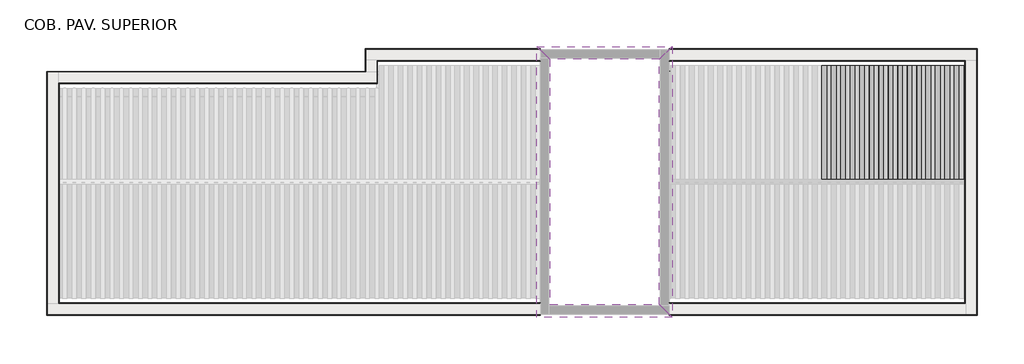
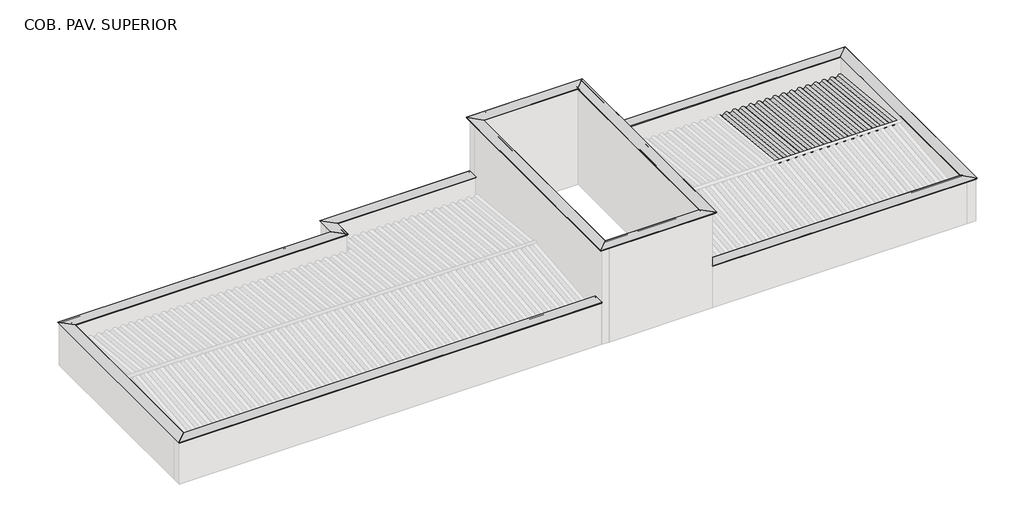
# One storey, part 7 of 7: 23 beams, 8 columns, 4 proxies.
"""IFC4 building model written with IfcOpenShell, lengths in millimetres."""

import ifcopenshell
import ifcopenshell.guid

model = None  # the IFC model being written
_history = None  # IfcOwnerHistory: only IFC2X3 demands one
_inside = {}  # id of a spatial element -> (the spatial element, [elements in it])
_under = {}  # id of a project, library or spatial element -> (it, [spatial elements below it])
_declared = {}  # id of a project -> (the project, [libraries it declares])
_typed = {}  # id of a type object -> (the type object, [elements of that type])
_made_of = {}  # id of a material, layer set ... -> (it, [elements and type objects made of it])


def new_model(schema):
    """Start an empty IFC model of exactly this schema.

    Asked for "IFC4X3", IfcOpenShell would pick the latest addendum, in which some entities
    have other attributes; the version numbers below select the first issue.
    IFC2X3 requires an IfcOwnerHistory on every rooted entity: one is made here for all.
    """
    global model, _history
    if schema == "IFC4X3":
        model = ifcopenshell.file(schema_version=(4, 3, 0, 0))
    else:
        model = ifcopenshell.file(schema=schema)
    _inside.clear()
    _under.clear()
    _declared.clear()
    _typed.clear()
    _made_of.clear()
    _history = None
    if model.schema == "IFC2X3":
        org = make("IfcOrganization", Name="unknown")
        user = make(
            "IfcPersonAndOrganization",
            ThePerson=make("IfcPerson", FamilyName="unknown"),
            TheOrganization=org,
        )
        app = make(
            "IfcApplication",
            ApplicationDeveloper=org,
            Version="unknown",
            ApplicationFullName="unknown",
            ApplicationIdentifier="unknown",
        )
        _history = make(
            "IfcOwnerHistory",
            OwningUser=user,
            OwningApplication=app,
            ChangeAction="ADDED",
            CreationDate=0,
        )
    return model


def make(cls, **values):
    """One entity of the class cls with the attributes given. An attribute that is None is left unset."""
    return model.create_entity(
        cls, **{name: value for name, value in values.items() if value is not None}
    )


def rooted(cls, **values):
    """An entity with a GlobalId (a new one), such as an element, a storey or a relation."""
    return make(cls, GlobalId=ifcopenshell.guid.new(), OwnerHistory=_history, **values)


def si_unit(unit_type, name, prefix=None):
    """IfcSIUnit, for example si_unit("LENGTHUNIT", "METRE", prefix="MILLI")."""
    return make("IfcSIUnit", UnitType=unit_type, Prefix=prefix, Name=name)


def assignment(units):
    """IfcUnitAssignment: the units of a project."""
    return None if units is None else make("IfcUnitAssignment", Units=units)


def point(xyz):
    """IfcCartesianPoint."""
    return None if xyz is None else make("IfcCartesianPoint", Coordinates=xyz)


def direction(xyz):
    """IfcDirection."""
    return None if xyz is None else make("IfcDirection", DirectionRatios=xyz)


def frame(location, z_axis=None, x_axis=None):
    """IfcAxis2Placement3D, a coordinate frame: its origin and axes. An axis left out is left unset."""
    return make(
        "IfcAxis2Placement3D",
        Location=point(location),
        Axis=direction(z_axis),
        RefDirection=direction(x_axis),
    )


def frame_2d(location, x_axis=None):
    """IfcAxis2Placement2D, a coordinate frame in the plane: its origin and x axis."""
    return make(
        "IfcAxis2Placement2D", Location=point(location), RefDirection=direction(x_axis)
    )


def origin():
    """The frame at (0, 0, 0) with its axes left unset."""
    return frame((0.0, 0.0, 0.0))


def place(relative_to, where):
    """IfcLocalPlacement: puts the frame where relative to a parent placement (None: the world)."""
    return make(
        "IfcLocalPlacement", PlacementRelTo=relative_to, RelativePlacement=where
    )


def context(
    kind, dimensions, precision=None, world=None, true_north=None, identifier=None
):
    """IfcGeometricRepresentationContext, for example the 3D "Model" context."""
    return make(
        "IfcGeometricRepresentationContext",
        ContextIdentifier=identifier,
        ContextType=kind,
        CoordinateSpaceDimension=dimensions,
        Precision=precision,
        WorldCoordinateSystem=world,
        TrueNorth=true_north,
    )


def project(units=None, contexts=None):
    """IfcProject with its units and contexts."""
    return rooted(
        "IfcProject",
        Name="project",
        RepresentationContexts=contexts,
        UnitsInContext=assignment(units),
    )


def spatial(cls, under=None, at=None, **own):
    """A site, building, storey or space (cls), placed at a placement, below another one or the project."""
    s = rooted(cls, ObjectPlacement=at, **own)
    if under is not None:
        _under.setdefault(under.id(), (under, []))[1].append(s)
    return s


def polyline(points):
    """IfcPolyline through the points."""
    return make("IfcPolyline", Points=[point(p) for p in points])


def circle_curve(where, radius):
    """IfcCircle in the frame where."""
    return make("IfcCircle", Position=where, Radius=radius)


def trimmed(basis, trim1, trim2, sense, master):
    """IfcTrimmedCurve: the piece of a basis curve between two trims."""
    return make(
        "IfcTrimmedCurve",
        BasisCurve=basis,
        Trim1=trim1,
        Trim2=trim2,
        SenseAgreement=sense,
        MasterRepresentation=master,
    )


def segment(curve, same_sense, transition):
    """IfcCompositeCurveSegment."""
    return make(
        "IfcCompositeCurveSegment",
        Transition=transition,
        SameSense=same_sense,
        ParentCurve=curve,
    )


def composite_curve(segments, self_intersect=None):
    """IfcCompositeCurve: segments joined end to end."""
    return make("IfcCompositeCurve", Segments=segments, SelfIntersect=self_intersect)


def outline(outer, holes=None, kind="AREA"):
    """IfcArbitraryClosedProfileDef: a profile drawn as a closed curve; with holes, ...WithVoids."""
    if holes is None:
        return make("IfcArbitraryClosedProfileDef", ProfileType=kind, OuterCurve=outer)
    return make(
        "IfcArbitraryProfileDefWithVoids",
        ProfileType=kind,
        OuterCurve=outer,
        InnerCurves=holes,
    )


def extrude(swept, where, along, depth):
    """IfcExtrudedAreaSolid: the profile swept, set in the frame where, extruded along a direction by depth."""
    return make(
        "IfcExtrudedAreaSolid",
        SweptArea=swept,
        Position=where,
        ExtrudedDirection=direction(along),
        Depth=depth,
    )


def faces_of(points, faces, orient=None, outer=None):
    """IfcFace entities. A face is a list of loops; a loop is a list of indices into points, from 0.

    orient and outer hold one flag for each loop. By default every Orientation is true, the
    first loop of a face is its IfcFaceOuterBound and the others are IfcFaceBound.
    """
    made = []
    for i, loops in enumerate(faces):
        bounds = []
        for j, loop in enumerate(loops):
            is_outer = j == 0 if outer is None else outer[i][j]
            bounds.append(
                make(
                    "IfcFaceOuterBound" if is_outer else "IfcFaceBound",
                    Bound=make("IfcPolyLoop", Polygon=[points[k] for k in loop]),
                    Orientation=True if orient is None else orient[i][j],
                )
            )
        made.append(make("IfcFace", Bounds=bounds))
    return made


def faceted_brep(points, faces, orient=None, outer=None, voids=None):
    """IfcFacetedBrep: a solid bounded by flat faces; with voids (closed shells), ...WithVoids."""
    shared = [point(p) for p in points]
    hull = make("IfcClosedShell", CfsFaces=faces_of(shared, faces, orient, outer))
    if voids is None:
        return make("IfcFacetedBrep", Outer=hull)
    return make(
        "IfcFacetedBrepWithVoids",
        Outer=hull,
        Voids=[
            make(cls, CfsFaces=faces_of(shared, fs, o, b)) for cls, fs, o, b in voids
        ],
    )


def shape(context_of_items, identifier, shape_type, items):
    """IfcShapeRepresentation: the items that make up one representation, for example the "Body"."""
    return make(
        "IfcShapeRepresentation",
        ContextOfItems=context_of_items,
        RepresentationIdentifier=identifier,
        RepresentationType=shape_type,
        Items=items,
    )


def source(mapping_origin, context_of_items, identifier, shape_type, items):
    """IfcRepresentationMap: a shape defined once, which mapped items show again and again."""
    return make(
        "IfcRepresentationMap",
        MappingOrigin=mapping_origin,
        MappedRepresentation=shape(context_of_items, identifier, shape_type, items),
    )


def transform(
    local_origin,
    x_axis=None,
    y_axis=None,
    z_axis=None,
    scale=None,
    scale2=None,
    scale3=None,
    uniform=True,
):
    """IfcCartesianTransformationOperator3D, or its non-uniform kind. x_axis, y_axis, z_axis: its Axis1, 2, 3."""
    if uniform:
        return make(
            "IfcCartesianTransformationOperator3D",
            Axis1=direction(x_axis),
            Axis2=direction(y_axis),
            LocalOrigin=point(local_origin),
            Scale=scale,
            Axis3=direction(z_axis),
        )
    return make(
        "IfcCartesianTransformationOperator3DnonUniform",
        Axis1=direction(x_axis),
        Axis2=direction(y_axis),
        LocalOrigin=point(local_origin),
        Scale=scale,
        Axis3=direction(z_axis),
        Scale2=scale2,
        Scale3=scale3,
    )


def mapped(mapping_source, mapping_target):
    """IfcMappedItem: shows the shape of a source again, moved by a transform."""
    return make(
        "IfcMappedItem", MappingSource=mapping_source, MappingTarget=mapping_target
    )


def made_of(thing, what):
    """Note that an element or type object is made of a material, layer set ...; save() writes the relation."""
    if what is not None:
        _made_of.setdefault(what.id(), (what, []))[1].append(thing)
    return thing


def element(
    cls,
    number,
    at=None,
    inside=None,
    cuts=None,
    type_object=None,
    material=None,
    context=None,
    identifier="Body",
    shape_type=None,
    held_by="IfcProductDefinitionShape",
    body=None,
    shapes=None,
    **own,
):
    """One element of the class cls, such as IfcWall. Its Tag is "e" and its number.

    at: its placement. inside: the storey or other place that contains it. cuts: it is an
    opening in that element (IfcRelVoidsElement). A single representation is given by context,
    identifier, shape_type and body (its items); several are given by shapes. held_by: the class
    of the entity that holds the representations. save() writes the other relations.
    """
    e = rooted(cls, Tag="e%d" % number, ObjectPlacement=at, **own)
    if body is not None:
        shapes = [shape(context, identifier, shape_type, body)]
    if shapes is not None:
        e.Representation = make(held_by, Representations=shapes)
    if inside is not None:
        _inside.setdefault(inside.id(), (inside, []))[1].append(e)
    if cuts is not None:
        rooted(
            "IfcRelVoidsElement", RelatingBuildingElement=cuts, RelatedOpeningElement=e
        )
    if type_object is not None:
        _typed.setdefault(type_object.id(), (type_object, []))[1].append(e)
    return made_of(e, material)


def aggregate(whole, parts):
    """IfcRelAggregates: a whole, such as a stair, and the parts it consists of."""
    return rooted("IfcRelAggregates", RelatingObject=whole, RelatedObjects=parts)


def save(model, path):
    """Write the relations noted so far, then the file.

    IfcRelAggregates (storeys below a building ...), IfcRelContainedInSpatialStructure (elements
    in a storey), IfcRelDefinesByType, IfcRelAssociatesMaterial and IfcRelDeclares: one each for
    every whole, place, type object, material and project.
    """
    for whole, parts in _under.values():
        aggregate(whole, parts)
    for where, things in _inside.values():
        rooted(
            "IfcRelContainedInSpatialStructure",
            RelatedElements=things,
            RelatingStructure=where,
        )
    for kind, things in _typed.values():
        rooted("IfcRelDefinesByType", RelatedObjects=things, RelatingType=kind)
    for what, things in _made_of.values():
        rooted("IfcRelAssociatesMaterial", RelatedObjects=things, RelatingMaterial=what)
    for by, libraries in _declared.values():
        rooted("IfcRelDeclares", RelatingContext=by, RelatedDefinitions=libraries)
    model.write(path)


def column_d505325c(model_context):
    return source(origin(), model_context, "Body", "SweptSolid", [
        extrude(outline(polyline([(30.0, 80.0), (30.0, -80.0), (-30.0, -80.0), (-30.0, 80.0), (30.0, 80.0)])), frame((0.0, 0.0, 6710.0), z_axis=(0.0, 0.0, 1.0), x_axis=(1.0, 0.0, 0.0)), (0.0, 0.0, 1.0), 750.0),
    ])


def column_4db371bd(model_context):
    return source(origin(), model_context, "Body", "SweptSolid", [
        extrude(outline(polyline([(30.0, 80.0), (30.0, -80.0), (-30.0, -80.0), (-30.0, 80.0), (30.0, 80.0)])), frame((0.0, 0.0, 6710.0), z_axis=(0.0, 0.0, 1.0), x_axis=(1.0, 0.0, 0.0)), (0.0, 0.0, 1.0), 660.0),
    ])


def column_d0cf395a(model_context):
    return source(origin(), model_context, "Body", "SweptSolid", [
        extrude(outline(polyline([(30.0, 80.0), (30.0, -80.0), (-30.0, -80.0), (-30.0, 80.0), (30.0, 80.0)])), frame((0.0, 0.0, 6710.0), z_axis=(0.0, 0.0, 1.0), x_axis=(1.0, 0.0, 0.0)), (0.0, 0.0, 1.0), 520.0),
    ])


model = new_model("IFC4")

# Units and contexts
model_context = context("Model", 3, world=origin())
ifc_project = project(units=[si_unit("LENGTHUNIT", "METRE", prefix="MILLI")], contexts=[model_context])

# Site, building, storey
site = spatial("IfcSite", under=ifc_project)
building = spatial("IfcBuilding", under=site)
storey = spatial("IfcBuildingStorey", under=building, Name="COB. PAV. SUPERIOR", Elevation=6650.0)

# Beams
placement = place(None, origin())
element("IfcBeam", 1, ObjectType="Madeira de lei : Berço 6x12cm", at=placement, inside=storey, context=model_context, shape_type="SweptSolid", body=[
    extrude(outline(polyline([(9090.718693, -7711.5607799), (9090.718693, -7831.5607799), (7090.718693, -7831.5607799), (7090.718693, -7711.5607799), (9090.718693, -7711.5607799)])), frame((0.0, 0.0, 6650.0), z_axis=(0.0, 0.0, 1.0), x_axis=(1.0, 0.0, 0.0)), (0.0, 0.0, 1.0), 60.0),
])
element("IfcBeam", 2, ObjectType="Madeira de lei : Berço 6x12cm", at=placement, inside=storey, context=model_context, shape_type="SweptSolid", body=[
    extrude(outline(polyline([(10730.718693, -7711.5607799), (10730.718693, -7831.5607799), (9090.718693, -7831.5607799), (9090.718693, -7711.5607799), (10730.718693, -7711.5607799)])), frame((0.0, 0.0, 6650.0), z_axis=(0.0, 0.0, 1.0), x_axis=(1.0, 0.0, 0.0)), (0.0, 0.0, 1.0), 60.0),
])
element("IfcBeam", 3, ObjectType="Madeira de lei : Berço 6x12cm", at=placement, inside=storey, context=model_context, shape_type="SweptSolid", body=[
    extrude(outline(polyline([(9089.7186924, -6319.8711004), (9089.7186924, -6439.8711004), (7089.7186936, -6439.8711004), (7089.7186936, -6319.8711004), (9089.7186924, -6319.8711004)])), frame((0.0, 0.0, 6650.0), z_axis=(0.0, 0.0, 1.0), x_axis=(1.0, 0.0, 0.0)), (0.0, 0.0, 1.0), 60.0),
])
element("IfcBeam", 4, ObjectType="Madeira de lei : Berço 6x12cm", at=placement, inside=storey, context=model_context, shape_type="SweptSolid", body=[
    extrude(outline(polyline([(10729.718693, -6319.8711004), (10729.718693, -6439.8711004), (9089.7186936, -6439.8711004), (9089.7186936, -6319.8711004), (10729.718693, -6319.8711004)])), frame((0.0, 0.0, 6650.0), z_axis=(0.0, 0.0, 1.0), x_axis=(1.0, 0.0, 0.0)), (0.0, 0.0, 1.0), 60.0),
])
element("IfcBeam", 5, ObjectType="Madeira de lei : Berço 6x12cm", at=placement, inside=storey, context=model_context, shape_type="SweptSolid", body=[
    extrude(outline(polyline([(5089.7186924, -4899.3026908), (5089.7186924, -5019.3026908), (3089.718693, -5019.3026908), (3089.718693, -4899.3026908), (5089.7186924, -4899.3026908)])), frame((0.0, 0.0, 6650.0), z_axis=(0.0, 0.0, 1.0), x_axis=(1.0, 0.0, 0.0)), (0.0, 0.0, 1.0), 60.0),
])
element("IfcBeam", 6, ObjectType="Madeira de lei : Berço 6x12cm", at=placement, inside=storey, context=model_context, shape_type="SweptSolid", body=[
    extrude(outline(polyline([(7089.7186924, -4899.3026908), (7089.7186924, -5019.3026908), (5089.7186936, -5019.3026908), (5089.7186936, -4899.3026908), (7089.7186924, -4899.3026908)])), frame((0.0, 0.0, 6650.0), z_axis=(0.0, 0.0, 1.0), x_axis=(1.0, 0.0, 0.0)), (0.0, 0.0, 1.0), 60.0),
])
element("IfcBeam", 7, ObjectType="Madeira de lei : Berço 6x12cm", at=placement, inside=storey, context=model_context, shape_type="SweptSolid", body=[
    extrude(outline(polyline([(9089.7186924, -4899.3026908), (9089.7186924, -5019.3026908), (7089.7186936, -5019.3026908), (7089.7186936, -4899.3026908), (9089.7186924, -4899.3026908)])), frame((0.0, 0.0, 6650.0), z_axis=(0.0, 0.0, 1.0), x_axis=(1.0, 0.0, 0.0)), (0.0, 0.0, 1.0), 60.0),
])
element("IfcBeam", 8, ObjectType="Madeira de lei : Berço 6x12cm", at=placement, inside=storey, context=model_context, shape_type="SweptSolid", body=[
    extrude(outline(polyline([(10729.718693, -4899.3026908), (10729.718693, -5019.3026908), (9089.7186936, -5019.3026908), (9089.7186936, -4899.3026908), (10729.718693, -4899.3026908)])), frame((0.0, 0.0, 6650.0), z_axis=(0.0, 0.0, 1.0), x_axis=(1.0, 0.0, 0.0)), (0.0, 0.0, 1.0), 60.0),
])
element("IfcBeam", 9, ObjectType="Telha Ondulada : Fibrocimento", at=placement, inside=storey, context=model_context, shape_type="SweptSolid", body=[
    extrude(outline(composite_curve([segment(trimmed(circle_curve(frame_2d((-58.7002978, -53.2060539)), 66.7939461), [point((-29.3501489, 6.7939461))], [point((-29.3501489, -113.2060539))], False, "CARTESIAN"), True, "CONTINUOUS"), segment(polyline([(-29.3501489, -113.2060539), (-31.5472154, -108.7146289)]), True, "CONTINUOUS"), segment(trimmed(circle_curve(frame_2d((-58.7002978, -53.2060539)), 61.7939461), [point((-31.5472154, -108.7146289))], [point((-31.5472154, 2.3025211))], True, "CARTESIAN"), True, "CONTINUOUS"), segment(trimmed(circle_curve(frame_2d((0.0, 66.7939461)), 71.7939461), [point((-31.5472154, 2.3025211))], [point((-31.5472154, 131.2853711))], False, "CARTESIAN"), True, "CONTINUOUS"), segment(polyline([(-31.5472154, 131.2853711), (-29.3501489, 126.7939461)]), True, "CONTINUOUS"), segment(trimmed(circle_curve(frame_2d((0.0, 66.7939461)), 66.7939461), [point((-29.3501489, 126.7939461))], [point((-29.3501489, 6.7939461))], True, "CARTESIAN"), True, "CONTINUOUS")], self_intersect=False)), frame((7168.1156257, -4759.1621575, 7394.5315886), z_axis=(0.0, -0.9950371902099893, 0.09950371902099778), x_axis=(0.0, 0.09950371902099778, 0.9950371902099893)), (0.0, 0.0, 1.0), 3017.2387654),
])
element("IfcBeam", 10, ObjectType="Telha Ondulada : Fibrocimento", at=placement, inside=storey, context=model_context, shape_type="SweptSolid", body=[
    extrude(outline(composite_curve([segment(trimmed(circle_curve(frame_2d((-58.7002978, -53.2060539)), 66.7939461), [point((-29.3501489, 6.7939461))], [point((-29.3501489, -113.2060539))], False, "CARTESIAN"), True, "CONTINUOUS"), segment(polyline([(-29.3501489, -113.2060539), (-31.5472154, -108.7146289)]), True, "CONTINUOUS"), segment(trimmed(circle_curve(frame_2d((-58.7002978, -53.2060539)), 61.7939461), [point((-31.5472154, -108.7146289))], [point((-31.5472154, 2.3025211))], True, "CARTESIAN"), True, "CONTINUOUS"), segment(trimmed(circle_curve(frame_2d((0.0, 66.7939461)), 71.7939461), [point((-31.5472154, 2.3025211))], [point((-31.5472154, 131.2853711))], False, "CARTESIAN"), True, "CONTINUOUS"), segment(polyline([(-31.5472154, 131.2853711), (-29.3501489, 126.7939461)]), True, "CONTINUOUS"), segment(trimmed(circle_curve(frame_2d((0.0, 66.7939461)), 66.7939461), [point((-29.3501489, 126.7939461))], [point((-29.3501489, 6.7939461))], True, "CARTESIAN"), True, "CONTINUOUS")], self_intersect=False)), frame((7412.6156257, -4759.1621575, 7394.5315886), z_axis=(0.0, -0.9950371902099893, 0.09950371902099776), x_axis=(0.0, 0.09950371902099776, 0.9950371902099893)), (0.0, 0.0, 1.0), 3017.2387654),
])
element("IfcBeam", 11, ObjectType="Telha Ondulada : Fibrocimento", at=placement, inside=storey, context=model_context, shape_type="SweptSolid", body=[
    extrude(outline(composite_curve([segment(trimmed(circle_curve(frame_2d((-58.7002978, -53.2060539)), 66.7939461), [point((-29.3501489, 6.7939461))], [point((-29.3501489, -113.2060539))], False, "CARTESIAN"), True, "CONTINUOUS"), segment(polyline([(-29.3501489, -113.2060539), (-31.5472154, -108.7146289)]), True, "CONTINUOUS"), segment(trimmed(circle_curve(frame_2d((-58.7002978, -53.2060539)), 61.7939461), [point((-31.5472154, -108.7146289))], [point((-31.5472154, 2.3025211))], True, "CARTESIAN"), True, "CONTINUOUS"), segment(trimmed(circle_curve(frame_2d((0.0, 66.7939461)), 71.7939461), [point((-31.5472154, 2.3025211))], [point((-31.5472154, 131.2853711))], False, "CARTESIAN"), True, "CONTINUOUS"), segment(polyline([(-31.5472154, 131.2853711), (-29.3501489, 126.7939461)]), True, "CONTINUOUS"), segment(trimmed(circle_curve(frame_2d((0.0, 66.7939461)), 66.7939461), [point((-29.3501489, 126.7939461))], [point((-29.3501489, 6.7939461))], True, "CARTESIAN"), True, "CONTINUOUS")], self_intersect=False)), frame((7657.1156257, -4759.1621575, 7394.5315886), z_axis=(0.0, -0.9950371902099893, 0.09950371902099775), x_axis=(0.0, 0.09950371902099775, 0.9950371902099893)), (0.0, 0.0, 1.0), 3017.2387654),
])
element("IfcBeam", 12, ObjectType="Telha Ondulada : Fibrocimento", at=placement, inside=storey, context=model_context, shape_type="SweptSolid", body=[
    extrude(outline(composite_curve([segment(trimmed(circle_curve(frame_2d((-58.7002978, -53.2060539)), 66.7939461), [point((-29.3501489, 6.7939461))], [point((-29.3501489, -113.2060539))], False, "CARTESIAN"), True, "CONTINUOUS"), segment(polyline([(-29.3501489, -113.2060539), (-31.5472154, -108.7146289)]), True, "CONTINUOUS"), segment(trimmed(circle_curve(frame_2d((-58.7002978, -53.2060539)), 61.7939461), [point((-31.5472154, -108.7146289))], [point((-31.5472154, 2.3025211))], True, "CARTESIAN"), True, "CONTINUOUS"), segment(trimmed(circle_curve(frame_2d((0.0, 66.7939461)), 71.7939461), [point((-31.5472154, 2.3025211))], [point((-31.5472154, 131.2853711))], False, "CARTESIAN"), True, "CONTINUOUS"), segment(polyline([(-31.5472154, 131.2853711), (-29.3501489, 126.7939461)]), True, "CONTINUOUS"), segment(trimmed(circle_curve(frame_2d((0.0, 66.7939461)), 66.7939461), [point((-29.3501489, 126.7939461))], [point((-29.3501489, 6.7939461))], True, "CARTESIAN"), True, "CONTINUOUS")], self_intersect=False)), frame((7901.6156257, -4759.1621575, 7394.5315886), z_axis=(0.0, -0.9950371902099893, 0.09950371902099778), x_axis=(0.0, 0.09950371902099778, 0.9950371902099893)), (0.0, 0.0, 1.0), 3017.2387654),
])
element("IfcBeam", 13, ObjectType="Telha Ondulada : Fibrocimento", at=placement, inside=storey, context=model_context, shape_type="SweptSolid", body=[
    extrude(outline(composite_curve([segment(trimmed(circle_curve(frame_2d((-58.7002978, -53.2060539)), 66.7939461), [point((-29.3501489, 6.7939461))], [point((-29.3501489, -113.2060539))], False, "CARTESIAN"), True, "CONTINUOUS"), segment(polyline([(-29.3501489, -113.2060539), (-31.5472154, -108.7146289)]), True, "CONTINUOUS"), segment(trimmed(circle_curve(frame_2d((-58.7002978, -53.2060539)), 61.7939461), [point((-31.5472154, -108.7146289))], [point((-31.5472154, 2.3025211))], True, "CARTESIAN"), True, "CONTINUOUS"), segment(trimmed(circle_curve(frame_2d((0.0, 66.7939461)), 71.7939461), [point((-31.5472154, 2.3025211))], [point((-31.5472154, 131.2853711))], False, "CARTESIAN"), True, "CONTINUOUS"), segment(polyline([(-31.5472154, 131.2853711), (-29.3501489, 126.7939461)]), True, "CONTINUOUS"), segment(trimmed(circle_curve(frame_2d((0.0, 66.7939461)), 66.7939461), [point((-29.3501489, 126.7939461))], [point((-29.3501489, 6.7939461))], True, "CARTESIAN"), True, "CONTINUOUS")], self_intersect=False)), frame((8146.1156257, -4759.1621575, 7394.5315886), z_axis=(0.0, -0.9950371902099893, 0.09950371902099776), x_axis=(0.0, 0.09950371902099776, 0.9950371902099893)), (0.0, 0.0, 1.0), 3017.2387654),
])
element("IfcBeam", 14, ObjectType="Telha Ondulada : Fibrocimento", at=placement, inside=storey, context=model_context, shape_type="SweptSolid", body=[
    extrude(outline(composite_curve([segment(trimmed(circle_curve(frame_2d((-58.7002978, -53.2060539)), 66.7939461), [point((-29.3501489, 6.7939461))], [point((-29.3501489, -113.2060539))], False, "CARTESIAN"), True, "CONTINUOUS"), segment(polyline([(-29.3501489, -113.2060539), (-31.5472154, -108.7146289)]), True, "CONTINUOUS"), segment(trimmed(circle_curve(frame_2d((-58.7002978, -53.2060539)), 61.7939461), [point((-31.5472154, -108.7146289))], [point((-31.5472154, 2.3025211))], True, "CARTESIAN"), True, "CONTINUOUS"), segment(trimmed(circle_curve(frame_2d((0.0, 66.7939461)), 71.7939461), [point((-31.5472154, 2.3025211))], [point((-31.5472154, 131.2853711))], False, "CARTESIAN"), True, "CONTINUOUS"), segment(polyline([(-31.5472154, 131.2853711), (-29.3501489, 126.7939461)]), True, "CONTINUOUS"), segment(trimmed(circle_curve(frame_2d((0.0, 66.7939461)), 66.7939461), [point((-29.3501489, 126.7939461))], [point((-29.3501489, 6.7939461))], True, "CARTESIAN"), True, "CONTINUOUS")], self_intersect=False)), frame((8390.6156257, -4759.1621575, 7394.5315886), z_axis=(0.0, -0.9950371902099893, 0.09950371902099776), x_axis=(0.0, 0.09950371902099776, 0.9950371902099893)), (0.0, 0.0, 1.0), 3017.2387654),
])
element("IfcBeam", 15, ObjectType="Telha Ondulada : Fibrocimento", at=placement, inside=storey, context=model_context, shape_type="SweptSolid", body=[
    extrude(outline(composite_curve([segment(trimmed(circle_curve(frame_2d((-58.7002978, -53.2060539)), 66.7939461), [point((-29.3501489, 6.7939461))], [point((-29.3501489, -113.2060539))], False, "CARTESIAN"), True, "CONTINUOUS"), segment(polyline([(-29.3501489, -113.2060539), (-31.5472154, -108.7146289)]), True, "CONTINUOUS"), segment(trimmed(circle_curve(frame_2d((-58.7002978, -53.2060539)), 61.7939461), [point((-31.5472154, -108.7146289))], [point((-31.5472154, 2.3025211))], True, "CARTESIAN"), True, "CONTINUOUS"), segment(trimmed(circle_curve(frame_2d((0.0, 66.7939461)), 71.7939461), [point((-31.5472154, 2.3025211))], [point((-31.5472154, 131.2853711))], False, "CARTESIAN"), True, "CONTINUOUS"), segment(polyline([(-31.5472154, 131.2853711), (-29.3501489, 126.7939461)]), True, "CONTINUOUS"), segment(trimmed(circle_curve(frame_2d((0.0, 66.7939461)), 66.7939461), [point((-29.3501489, 126.7939461))], [point((-29.3501489, 6.7939461))], True, "CARTESIAN"), True, "CONTINUOUS")], self_intersect=False)), frame((8635.1156257, -4759.1621575, 7394.5315886), z_axis=(0.0, -0.9950371902099893, 0.09950371902099778), x_axis=(0.0, 0.09950371902099778, 0.9950371902099893)), (0.0, 0.0, 1.0), 3017.2387654),
])
element("IfcBeam", 16, ObjectType="Telha Ondulada : Fibrocimento", at=placement, inside=storey, context=model_context, shape_type="SweptSolid", body=[
    extrude(outline(composite_curve([segment(trimmed(circle_curve(frame_2d((-58.7002978, -53.2060539)), 66.7939461), [point((-29.3501489, 6.7939461))], [point((-29.3501489, -113.2060539))], False, "CARTESIAN"), True, "CONTINUOUS"), segment(polyline([(-29.3501489, -113.2060539), (-31.5472154, -108.7146289)]), True, "CONTINUOUS"), segment(trimmed(circle_curve(frame_2d((-58.7002978, -53.2060539)), 61.7939461), [point((-31.5472154, -108.7146289))], [point((-31.5472154, 2.3025211))], True, "CARTESIAN"), True, "CONTINUOUS"), segment(trimmed(circle_curve(frame_2d((0.0, 66.7939461)), 71.7939461), [point((-31.5472154, 2.3025211))], [point((-31.5472154, 131.2853711))], False, "CARTESIAN"), True, "CONTINUOUS"), segment(polyline([(-31.5472154, 131.2853711), (-29.3501489, 126.7939461)]), True, "CONTINUOUS"), segment(trimmed(circle_curve(frame_2d((0.0, 66.7939461)), 66.7939461), [point((-29.3501489, 126.7939461))], [point((-29.3501489, 6.7939461))], True, "CARTESIAN"), True, "CONTINUOUS")], self_intersect=False)), frame((8879.6156257, -4759.1621575, 7394.5315886), z_axis=(0.0, -0.9950371902099893, 0.09950371902099778), x_axis=(0.0, 0.09950371902099778, 0.9950371902099893)), (0.0, 0.0, 1.0), 3017.2387654),
])
element("IfcBeam", 17, ObjectType="Telha Ondulada : Fibrocimento", at=placement, inside=storey, context=model_context, shape_type="SweptSolid", body=[
    extrude(outline(composite_curve([segment(trimmed(circle_curve(frame_2d((-58.7002978, -53.2060539)), 66.7939461), [point((-29.3501489, 6.7939461))], [point((-29.3501489, -113.2060539))], False, "CARTESIAN"), True, "CONTINUOUS"), segment(polyline([(-29.3501489, -113.2060539), (-31.5472154, -108.7146289)]), True, "CONTINUOUS"), segment(trimmed(circle_curve(frame_2d((-58.7002978, -53.2060539)), 61.7939461), [point((-31.5472154, -108.7146289))], [point((-31.5472154, 2.3025211))], True, "CARTESIAN"), True, "CONTINUOUS"), segment(trimmed(circle_curve(frame_2d((0.0, 66.7939461)), 71.7939461), [point((-31.5472154, 2.3025211))], [point((-31.5472154, 131.2853711))], False, "CARTESIAN"), True, "CONTINUOUS"), segment(polyline([(-31.5472154, 131.2853711), (-29.3501489, 126.7939461)]), True, "CONTINUOUS"), segment(trimmed(circle_curve(frame_2d((0.0, 66.7939461)), 66.7939461), [point((-29.3501489, 126.7939461))], [point((-29.3501489, 6.7939461))], True, "CARTESIAN"), True, "CONTINUOUS")], self_intersect=False)), frame((9124.1156257, -4759.1621575, 7394.5315886), z_axis=(0.0, -0.9950371902099893, 0.09950371902099776), x_axis=(0.0, 0.09950371902099776, 0.9950371902099893)), (0.0, 0.0, 1.0), 3017.2387654),
])
element("IfcBeam", 18, ObjectType="Telha Ondulada : Fibrocimento", at=placement, inside=storey, context=model_context, shape_type="SweptSolid", body=[
    extrude(outline(composite_curve([segment(trimmed(circle_curve(frame_2d((-58.7002978, -53.2060539)), 66.7939461), [point((-29.3501489, 6.7939461))], [point((-29.3501489, -113.2060539))], False, "CARTESIAN"), True, "CONTINUOUS"), segment(polyline([(-29.3501489, -113.2060539), (-31.5472154, -108.7146289)]), True, "CONTINUOUS"), segment(trimmed(circle_curve(frame_2d((-58.7002978, -53.2060539)), 61.7939461), [point((-31.5472154, -108.7146289))], [point((-31.5472154, 2.3025211))], True, "CARTESIAN"), True, "CONTINUOUS"), segment(trimmed(circle_curve(frame_2d((0.0, 66.7939461)), 71.7939461), [point((-31.5472154, 2.3025211))], [point((-31.5472154, 131.2853711))], False, "CARTESIAN"), True, "CONTINUOUS"), segment(polyline([(-31.5472154, 131.2853711), (-29.3501489, 126.7939461)]), True, "CONTINUOUS"), segment(trimmed(circle_curve(frame_2d((0.0, 66.7939461)), 66.7939461), [point((-29.3501489, 126.7939461))], [point((-29.3501489, 6.7939461))], True, "CARTESIAN"), True, "CONTINUOUS")], self_intersect=False)), frame((9368.6156257, -4759.1621575, 7394.5315886), z_axis=(0.0, -0.9950371902099893, 0.09950371902099776), x_axis=(0.0, 0.09950371902099776, 0.9950371902099893)), (0.0, 0.0, 1.0), 3017.2387654),
])
element("IfcBeam", 19, ObjectType="Telha Ondulada : Fibrocimento", at=placement, inside=storey, context=model_context, shape_type="SweptSolid", body=[
    extrude(outline(composite_curve([segment(trimmed(circle_curve(frame_2d((-58.7002978, -53.2060539)), 66.7939461), [point((-29.3501489, 6.7939461))], [point((-29.3501489, -113.2060539))], False, "CARTESIAN"), True, "CONTINUOUS"), segment(polyline([(-29.3501489, -113.2060539), (-31.5472154, -108.7146289)]), True, "CONTINUOUS"), segment(trimmed(circle_curve(frame_2d((-58.7002978, -53.2060539)), 61.7939461), [point((-31.5472154, -108.7146289))], [point((-31.5472154, 2.3025211))], True, "CARTESIAN"), True, "CONTINUOUS"), segment(trimmed(circle_curve(frame_2d((0.0, 66.7939461)), 71.7939461), [point((-31.5472154, 2.3025211))], [point((-31.5472154, 131.2853711))], False, "CARTESIAN"), True, "CONTINUOUS"), segment(polyline([(-31.5472154, 131.2853711), (-29.3501489, 126.7939461)]), True, "CONTINUOUS"), segment(trimmed(circle_curve(frame_2d((0.0, 66.7939461)), 66.7939461), [point((-29.3501489, 126.7939461))], [point((-29.3501489, 6.7939461))], True, "CARTESIAN"), True, "CONTINUOUS")], self_intersect=False)), frame((9613.1156257, -4759.1621575, 7394.5315886), z_axis=(0.0, -0.9950371902099893, 0.09950371902099775), x_axis=(0.0, 0.09950371902099775, 0.9950371902099893)), (0.0, 0.0, 1.0), 3017.2387654),
])
element("IfcBeam", 20, ObjectType="Telha Ondulada : Fibrocimento", at=placement, inside=storey, context=model_context, shape_type="SweptSolid", body=[
    extrude(outline(composite_curve([segment(trimmed(circle_curve(frame_2d((-58.7002978, -53.2060539)), 66.7939461), [point((-29.3501489, 6.7939461))], [point((-29.3501489, -113.2060539))], False, "CARTESIAN"), True, "CONTINUOUS"), segment(polyline([(-29.3501489, -113.2060539), (-31.5472154, -108.7146289)]), True, "CONTINUOUS"), segment(trimmed(circle_curve(frame_2d((-58.7002978, -53.2060539)), 61.7939461), [point((-31.5472154, -108.7146289))], [point((-31.5472154, 2.3025211))], True, "CARTESIAN"), True, "CONTINUOUS"), segment(trimmed(circle_curve(frame_2d((0.0, 66.7939461)), 71.7939461), [point((-31.5472154, 2.3025211))], [point((-31.5472154, 131.2853711))], False, "CARTESIAN"), True, "CONTINUOUS"), segment(polyline([(-31.5472154, 131.2853711), (-29.3501489, 126.7939461)]), True, "CONTINUOUS"), segment(trimmed(circle_curve(frame_2d((0.0, 66.7939461)), 66.7939461), [point((-29.3501489, 126.7939461))], [point((-29.3501489, 6.7939461))], True, "CARTESIAN"), True, "CONTINUOUS")], self_intersect=False)), frame((9857.6156257, -4759.1621575, 7394.5315886), z_axis=(0.0, -0.9950371902099893, 0.09950371902099778), x_axis=(0.0, 0.09950371902099778, 0.9950371902099893)), (0.0, 0.0, 1.0), 3017.2387654),
])
element("IfcBeam", 21, ObjectType="Telha Ondulada : Fibrocimento", at=placement, inside=storey, context=model_context, shape_type="SweptSolid", body=[
    extrude(outline(composite_curve([segment(trimmed(circle_curve(frame_2d((-58.7002978, -53.2060539)), 66.7939461), [point((-29.3501489, 6.7939461))], [point((-29.3501489, -113.2060539))], False, "CARTESIAN"), True, "CONTINUOUS"), segment(polyline([(-29.3501489, -113.2060539), (-31.5472154, -108.7146289)]), True, "CONTINUOUS"), segment(trimmed(circle_curve(frame_2d((-58.7002978, -53.2060539)), 61.7939461), [point((-31.5472154, -108.7146289))], [point((-31.5472154, 2.3025211))], True, "CARTESIAN"), True, "CONTINUOUS"), segment(trimmed(circle_curve(frame_2d((0.0, 66.7939461)), 71.7939461), [point((-31.5472154, 2.3025211))], [point((-31.5472154, 131.2853711))], False, "CARTESIAN"), True, "CONTINUOUS"), segment(polyline([(-31.5472154, 131.2853711), (-29.3501489, 126.7939461)]), True, "CONTINUOUS"), segment(trimmed(circle_curve(frame_2d((0.0, 66.7939461)), 66.7939461), [point((-29.3501489, 126.7939461))], [point((-29.3501489, 6.7939461))], True, "CARTESIAN"), True, "CONTINUOUS")], self_intersect=False)), frame((10102.1156257, -4759.1621575, 7394.5315886), z_axis=(0.0, -0.9950371902099893, 0.09950371902099776), x_axis=(0.0, 0.09950371902099776, 0.9950371902099893)), (0.0, 0.0, 1.0), 3017.2387654),
])
element("IfcBeam", 22, ObjectType="Telha Ondulada : Fibrocimento", at=placement, inside=storey, context=model_context, shape_type="SweptSolid", body=[
    extrude(outline(composite_curve([segment(trimmed(circle_curve(frame_2d((-58.7002978, -53.2060539)), 66.7939461), [point((-29.3501489, 6.7939461))], [point((-29.3501489, -113.2060539))], False, "CARTESIAN"), True, "CONTINUOUS"), segment(polyline([(-29.3501489, -113.2060539), (-31.5472154, -108.7146289)]), True, "CONTINUOUS"), segment(trimmed(circle_curve(frame_2d((-58.7002978, -53.2060539)), 61.7939461), [point((-31.5472154, -108.7146289))], [point((-31.5472154, 2.3025211))], True, "CARTESIAN"), True, "CONTINUOUS"), segment(trimmed(circle_curve(frame_2d((0.0, 66.7939461)), 71.7939461), [point((-31.5472154, 2.3025211))], [point((-31.5472154, 131.2853711))], False, "CARTESIAN"), True, "CONTINUOUS"), segment(polyline([(-31.5472154, 131.2853711), (-29.3501489, 126.7939461)]), True, "CONTINUOUS"), segment(trimmed(circle_curve(frame_2d((0.0, 66.7939461)), 66.7939461), [point((-29.3501489, 126.7939461))], [point((-29.3501489, 6.7939461))], True, "CARTESIAN"), True, "CONTINUOUS")], self_intersect=False)), frame((10346.6156257, -4759.1621575, 7394.5315886), z_axis=(0.0, -0.9950371902099893, 0.09950371902099776), x_axis=(0.0, 0.09950371902099776, 0.9950371902099893)), (0.0, 0.0, 1.0), 3017.2387654),
])
element("IfcBeam", 23, ObjectType="Telha Ondulada : Fibrocimento", at=placement, inside=storey, context=model_context, shape_type="SweptSolid", body=[
    extrude(outline(composite_curve([segment(trimmed(circle_curve(frame_2d((-58.7002978, -53.2060539)), 66.7939461), [point((-29.3501489, 6.7939461))], [point((-29.3501489, -113.2060539))], False, "CARTESIAN"), True, "CONTINUOUS"), segment(polyline([(-29.3501489, -113.2060539), (-31.5472154, -108.7146289)]), True, "CONTINUOUS"), segment(trimmed(circle_curve(frame_2d((-58.7002978, -53.2060539)), 61.7939461), [point((-31.5472154, -108.7146289))], [point((-31.5472154, 2.3025211))], True, "CARTESIAN"), True, "CONTINUOUS"), segment(trimmed(circle_curve(frame_2d((0.0, 66.7939461)), 71.7939461), [point((-31.5472154, 2.3025211))], [point((-31.5472154, 131.2853711))], False, "CARTESIAN"), True, "CONTINUOUS"), segment(polyline([(-31.5472154, 131.2853711), (-29.3501489, 126.7939461)]), True, "CONTINUOUS"), segment(trimmed(circle_curve(frame_2d((0.0, 66.7939461)), 66.7939461), [point((-29.3501489, 126.7939461))], [point((-29.3501489, 6.7939461))], True, "CARTESIAN"), True, "CONTINUOUS")], self_intersect=False)), frame((10591.1156257, -4759.1621575, 7394.5315886), z_axis=(0.0, -0.9950371902099893, 0.09950371902099778), x_axis=(0.0, 0.09950371902099778, 0.9950371902099893)), (0.0, 0.0, 1.0), 3017.2387654),
])

# Proxies
element("IfcBuildingElementProxy", 24, Name=".CC_RUFO_PINGADEIRA_27 cm", ObjectType=".CC_RUFO_PINGADEIRA_27 cm", at=placement, inside=storey, context=model_context, shape_type="Brep", body=[
    faceted_brep([(-4754.5024445, -4334.3488472, 7826.6820963), (-4747.4313766, -4341.419915, 7833.7531641), (-4747.4313766, -4341.419915, 7836.5815912), (-4754.0054581, -4334.8458336, 7830.0075098), (-4769.952748, -4318.8985437, 7860.0), (-4443.6098659, -4645.2414257, 7860.0), (-4459.5571559, -4629.2941358, 7830.0075098), (-4466.1312373, -4622.7200544, 7836.5815912), (-4466.1312373, -4622.7200544, 7833.7531641), (-4459.0601695, -4629.7911222, 7826.6820963), (-4440.281307, -4648.5699847, 7862.0), (-4773.281307, -4315.5699847, 7862.0), (-243.281307, -4334.3488472, 7826.6820963), (-243.281307, -4315.5699847, 7862.0), (-243.281307, -4648.5699847, 7862.0), (-243.281307, -4629.7911222, 7826.6820963), (-243.281307, -4622.7200544, 7833.7531641), (-243.281307, -4622.7200544, 7836.5815912), (-243.281307, -4629.2941358, 7830.0075098), (-243.281307, -4645.2414257, 7860.0), (-243.281307, -4318.8985437, 7860.0), (-243.281307, -4334.8458336, 7830.0075098), (-243.281307, -4341.419915, 7836.5815912), (-243.281307, -4341.419915, 7833.7531641)], [[[0, 1, 2, 3, 4, 5, 6, 7, 8, 9, 10, 11]], [[12, 13, 14, 15, 16, 17, 18, 19, 20, 21, 22, 23]], [[1, 0, 12, 23]], [[2, 1, 23, 22]], [[3, 2, 22, 21]], [[4, 3, 21, 20]], [[5, 4, 20, 19]], [[6, 5, 19, 18]], [[7, 6, 18, 17]], [[8, 7, 17, 16]], [[9, 8, 16, 15]], [[10, 9, 15, 14]], [[11, 10, 14, 13]], [[0, 11, 13, 12]]]),
    faceted_brep([(-4754.5024445, -4923.3488472, 7826.6820963), (-4747.4313766, -4930.419915, 7833.7531641), (-4747.4313766, -4930.419915, 7836.5815912), (-4754.0054581, -4923.8458336, 7830.0075098), (-4769.952748, -4907.8985437, 7860.0), (-4443.6098659, -5234.2414257, 7860.0), (-4459.5571559, -5218.2941358, 7830.0075098), (-4466.1312373, -5211.7200544, 7836.5815912), (-4466.1312373, -5211.7200544, 7833.7531641), (-4459.0601695, -5218.7911222, 7826.6820963), (-4440.281307, -5237.5699847, 7862.0), (-4773.281307, -4904.5699847, 7862.0), (-4754.5024445, -4334.3488472, 7826.6820963), (-4773.281307, -4315.5699847, 7862.0), (-4440.281307, -4648.5699847, 7862.0), (-4459.0601695, -4629.7911222, 7826.6820963), (-4466.1312373, -4622.7200544, 7833.7531641), (-4466.1312373, -4622.7200544, 7836.5815912), (-4459.5571559, -4629.2941358, 7830.0075098), (-4443.6098659, -4645.2414257, 7860.0), (-4769.952748, -4318.8985437, 7860.0), (-4754.0054581, -4334.8458336, 7830.0075098), (-4747.4313766, -4341.419915, 7836.5815912), (-4747.4313766, -4341.419915, 7833.7531641)], [[[0, 1, 2, 3, 4, 5, 6, 7, 8, 9, 10, 11]], [[12, 13, 14, 15, 16, 17, 18, 19, 20, 21, 22, 23]], [[1, 0, 12, 23]], [[2, 1, 23, 22]], [[3, 2, 22, 21]], [[4, 3, 21, 20]], [[5, 4, 20, 19]], [[6, 5, 19, 18]], [[7, 6, 18, 17]], [[8, 7, 17, 16]], [[9, 8, 16, 15]], [[10, 9, 15, 14]], [[11, 10, 14, 13]], [[0, 11, 13, 12]]]),
    faceted_brep([(-12982.5024444, -4923.3488472, 7826.6820963), (-12975.4313766, -4930.419915, 7833.7531641), (-12975.4313766, -4930.419915, 7836.5815912), (-12982.0054581, -4923.8458336, 7830.0075098), (-12997.952748, -4907.8985437, 7860.0), (-12671.6098659, -5234.2414257, 7860.0), (-12687.5571558, -5218.2941358, 7830.0075098), (-12694.1312373, -5211.7200544, 7836.5815912), (-12694.1312373, -5211.7200544, 7833.7531641), (-12687.0601695, -5218.7911222, 7826.6820963), (-12668.2813069, -5237.5699847, 7862.0), (-13001.2813069, -4904.5699847, 7862.0), (-4754.5024445, -4923.3488472, 7826.6820963), (-4773.281307, -4904.5699847, 7862.0), (-4440.281307, -5237.5699847, 7862.0), (-4459.0601695, -5218.7911222, 7826.6820963), (-4466.1312373, -5211.7200544, 7833.7531641), (-4466.1312373, -5211.7200544, 7836.5815912), (-4459.5571559, -5218.2941358, 7830.0075098), (-4443.6098659, -5234.2414257, 7860.0), (-4769.952748, -4907.8985437, 7860.0), (-4754.0054581, -4923.8458336, 7830.0075098), (-4747.4313766, -4930.419915, 7836.5815912), (-4747.4313766, -4930.419915, 7833.7531641)], [[[0, 1, 2, 3, 4, 5, 6, 7, 8, 9, 10, 11]], [[12, 13, 14, 15, 16, 17, 18, 19, 20, 21, 22, 23]], [[1, 0, 12, 23]], [[2, 1, 23, 22]], [[3, 2, 22, 21]], [[4, 3, 21, 20]], [[5, 4, 20, 19]], [[6, 5, 19, 18]], [[7, 6, 18, 17]], [[8, 7, 17, 16]], [[9, 8, 16, 15]], [[10, 9, 15, 14]], [[11, 10, 14, 13]], [[0, 11, 13, 12]]]),
    faceted_brep([(-12982.5024444, -11206.7911222, 7826.6820963), (-12975.4313766, -11199.7200544, 7833.7531641), (-12975.4313766, -11199.7200544, 7836.5815912), (-12982.0054581, -11206.2941358, 7830.0075098), (-12997.952748, -11222.2414257, 7860.0), (-12671.6098659, -10895.8985437, 7860.0), (-12687.5571558, -10911.8458336, 7830.0075098), (-12694.1312373, -10918.419915, 7836.5815912), (-12694.1312373, -10918.419915, 7833.7531641), (-12687.0601695, -10911.3488472, 7826.6820963), (-12668.2813069, -10892.5699847, 7862.0), (-13001.2813069, -11225.5699847, 7862.0), (-12982.5024444, -4923.3488472, 7826.6820963), (-13001.2813069, -4904.5699847, 7862.0), (-12668.2813069, -5237.5699847, 7862.0), (-12687.0601695, -5218.7911222, 7826.6820963), (-12694.1312373, -5211.7200544, 7833.7531641), (-12694.1312373, -5211.7200544, 7836.5815912), (-12687.5571558, -5218.2941358, 7830.0075098), (-12671.6098659, -5234.2414257, 7860.0), (-12997.952748, -4907.8985437, 7860.0), (-12982.0054581, -4923.8458336, 7830.0075098), (-12975.4313766, -4930.419915, 7836.5815912), (-12975.4313766, -4930.419915, 7833.7531641)], [[[0, 1, 2, 3, 4, 5, 6, 7, 8, 9, 10, 11]], [[12, 13, 14, 15, 16, 17, 18, 19, 20, 21, 22, 23]], [[1, 0, 12, 23]], [[2, 1, 23, 22]], [[3, 2, 22, 21]], [[4, 3, 21, 20]], [[5, 4, 20, 19]], [[6, 5, 19, 18]], [[7, 6, 18, 17]], [[8, 7, 17, 16]], [[9, 8, 16, 15]], [[10, 9, 15, 14]], [[11, 10, 14, 13]], [[0, 11, 13, 12]]]),
    faceted_brep([(-243.281307, -11206.7911222, 7826.6820963), (-243.281307, -11199.7200544, 7833.7531641), (-243.281307, -11199.7200544, 7836.5815912), (-243.281307, -11206.2941358, 7830.0075098), (-243.281307, -11222.2414257, 7860.0), (-243.281307, -10895.8985437, 7860.0), (-243.281307, -10911.8458336, 7830.0075098), (-243.281307, -10918.419915, 7836.5815912), (-243.281307, -10918.419915, 7833.7531641), (-243.281307, -10911.3488472, 7826.6820963), (-243.281307, -10892.5699847, 7862.0), (-243.281307, -11225.5699847, 7862.0), (-12982.5024444, -11206.7911222, 7826.6820963), (-13001.2813069, -11225.5699847, 7862.0), (-12668.2813069, -10892.5699847, 7862.0), (-12687.0601695, -10911.3488472, 7826.6820963), (-12694.1312373, -10918.419915, 7833.7531641), (-12694.1312373, -10918.419915, 7836.5815912), (-12687.5571558, -10911.8458336, 7830.0075098), (-12671.6098659, -10895.8985437, 7860.0), (-12997.952748, -11222.2414257, 7860.0), (-12982.0054581, -11206.2941358, 7830.0075098), (-12975.4313766, -11199.7200544, 7836.5815912), (-12975.4313766, -11199.7200544, 7833.7531641)], [[[0, 1, 2, 3, 4, 5, 6, 7, 8, 9, 10, 11]], [[12, 13, 14, 15, 16, 17, 18, 19, 20, 21, 22, 23]], [[1, 0, 12, 23]], [[2, 1, 23, 22]], [[3, 2, 22, 21]], [[4, 3, 21, 20]], [[5, 4, 20, 19]], [[6, 5, 19, 18]], [[7, 6, 18, 17]], [[8, 7, 17, 16]], [[9, 8, 16, 15]], [[10, 9, 15, 14]], [[11, 10, 14, 13]], [[0, 11, 13, 12]]]),
    faceted_brep([(11042.9398305, -11206.7911222, 7826.6820963), (11035.8687627, -11199.7200544, 7833.7531641), (11035.8687627, -11199.7200544, 7836.5815912), (11042.4428441, -11206.2941358, 7830.0075098), (11058.3901341, -11222.2414257, 7860.0), (10732.047252, -10895.8985437, 7860.0), (10747.9945419, -10911.8458336, 7830.0075098), (10754.5686234, -10918.419915, 7836.5815912), (10754.5686234, -10918.419915, 7833.7531641), (10747.4975555, -10911.3488472, 7826.6820963), (10728.718693, -10892.5699847, 7862.0), (11061.718693, -11225.5699847, 7862.0), (3090.718693, -11206.7911222, 7826.6820963), (3090.718693, -11225.5699847, 7862.0), (3090.718693, -10892.5699847, 7862.0), (3090.718693, -10911.3488472, 7826.6820963), (3090.718693, -10918.419915, 7833.7531641), (3090.718693, -10918.419915, 7836.5815912), (3090.718693, -10911.8458336, 7830.0075098), (3090.718693, -10895.8985437, 7860.0), (3090.718693, -11222.2414257, 7860.0), (3090.718693, -11206.2941358, 7830.0075098), (3090.718693, -11199.7200544, 7836.5815912), (3090.718693, -11199.7200544, 7833.7531641)], [[[0, 1, 2, 3, 4, 5, 6, 7, 8, 9, 10, 11]], [[12, 13, 14, 15, 16, 17, 18, 19, 20, 21, 22, 23]], [[1, 0, 12, 23]], [[2, 1, 23, 22]], [[3, 2, 22, 21]], [[4, 3, 21, 20]], [[5, 4, 20, 19]], [[6, 5, 19, 18]], [[7, 6, 18, 17]], [[8, 7, 17, 16]], [[9, 8, 16, 15]], [[10, 9, 15, 14]], [[11, 10, 14, 13]], [[0, 11, 13, 12]]]),
    faceted_brep([(11042.9398305, -4334.3304376, 7826.6820963), (11035.8687627, -4341.4015054, 7833.7531641), (11035.8687627, -4341.4015054, 7836.5815912), (11042.4428441, -4334.827424, 7830.0075098), (11058.3901341, -4318.8801341, 7860.0), (10732.047252, -4645.2230161, 7860.0), (10747.9945419, -4629.2757262, 7830.0075098), (10754.5686234, -4622.7016448, 7836.5815912), (10754.5686234, -4622.7016448, 7833.7531641), (10747.4975555, -4629.7727126, 7826.6820963), (10728.718693, -4648.5515751, 7862.0), (11061.718693, -4315.5515751, 7862.0), (11042.9398305, -11206.7911222, 7826.6820963), (11061.718693, -11225.5699847, 7862.0), (10728.718693, -10892.5699847, 7862.0), (10747.4975555, -10911.3488472, 7826.6820963), (10754.5686234, -10918.419915, 7833.7531641), (10754.5686234, -10918.419915, 7836.5815912), (10747.9945419, -10911.8458336, 7830.0075098), (10732.047252, -10895.8985437, 7860.0), (11058.3901341, -11222.2414257, 7860.0), (11042.4428441, -11206.2941358, 7830.0075098), (11035.8687627, -11199.7200544, 7836.5815912), (11035.8687627, -11199.7200544, 7833.7531641)], [[[0, 1, 2, 3, 4, 5, 6, 7, 8, 9, 10, 11]], [[12, 13, 14, 15, 16, 17, 18, 19, 20, 21, 22, 23]], [[1, 0, 12, 23]], [[2, 1, 23, 22]], [[3, 2, 22, 21]], [[4, 3, 21, 20]], [[5, 4, 20, 19]], [[6, 5, 19, 18]], [[7, 6, 18, 17]], [[8, 7, 17, 16]], [[9, 8, 16, 15]], [[10, 9, 15, 14]], [[11, 10, 14, 13]], [[0, 11, 13, 12]]]),
    faceted_brep([(3090.718693, -4334.3304376, 7826.6820963), (3090.718693, -4341.4015054, 7833.7531641), (3090.718693, -4341.4015054, 7836.5815912), (3090.718693, -4334.827424, 7830.0075098), (3090.718693, -4318.8801341, 7860.0), (3090.718693, -4645.2230161, 7860.0), (3090.718693, -4629.2757262, 7830.0075098), (3090.718693, -4622.7016448, 7836.5815912), (3090.718693, -4622.7016448, 7833.7531641), (3090.718693, -4629.7727126, 7826.6820963), (3090.718693, -4648.5515751, 7862.0), (3090.718693, -4315.5515751, 7862.0), (11042.9398305, -4334.3304376, 7826.6820963), (11061.718693, -4315.5515751, 7862.0), (10728.718693, -4648.5515751, 7862.0), (10747.4975555, -4629.7727126, 7826.6820963), (10754.5686234, -4622.7016448, 7833.7531641), (10754.5686234, -4622.7016448, 7836.5815912), (10747.9945419, -4629.2757262, 7830.0075098), (10732.047252, -4645.2230161, 7860.0), (11058.3901341, -4318.8801341, 7860.0), (11042.4428441, -4334.827424, 7830.0075098), (11035.8687627, -4341.4015054, 7836.5815912), (11035.8687627, -4341.4015054, 7833.7531641)], [[[0, 1, 2, 3, 4, 5, 6, 7, 8, 9, 10, 11]], [[12, 13, 14, 15, 16, 17, 18, 19, 20, 21, 22, 23]], [[1, 0, 12, 23]], [[2, 1, 23, 22]], [[3, 2, 22, 21]], [[4, 3, 21, 20]], [[5, 4, 20, 19]], [[6, 5, 19, 18]], [[7, 6, 18, 17]], [[8, 7, 17, 16]], [[9, 8, 16, 15]], [[10, 9, 15, 14]], [[11, 10, 14, 13]], [[0, 11, 13, 12]]]),
])
element("IfcBuildingElementProxy", 25, Name=".CC_RUFO_PINGADEIRA_27 cm", ObjectType=".CC_RUFO_PINGADEIRA_27 cm", at=placement, inside=storey, context=model_context, shape_type="Brep", body=[
    faceted_brep([(2857.4975555, -10962.3488472, 9526.6820963), (2838.718693, -10943.5699847, 9562.0), (3171.718693, -11276.5699847, 9562.0), (3152.9398305, -11257.7911222, 9526.6820963), (3145.8687627, -11250.7200544, 9533.7531641), (3145.8687627, -11250.7200544, 9536.5815912), (3152.4428441, -11257.2941358, 9530.0075098), (3168.3901341, -11273.2414257, 9560.0), (2842.047252, -10946.8985437, 9560.0), (2857.9945419, -10962.8458336, 9530.0075098), (2864.5686234, -10969.419915, 9536.5815912), (2864.5686234, -10969.419915, 9533.7531641), (-10.0601695, -10962.3488472, 9526.6820963), (-17.1312373, -10969.419915, 9533.7531641), (-17.1312373, -10969.419915, 9536.5815912), (-10.5571559, -10962.8458336, 9530.0075098), (5.3901341, -10946.8985437, 9560.0), (-320.952748, -11273.2414257, 9560.0), (-305.0054581, -11257.2941358, 9530.0075098), (-298.4313766, -11250.7200544, 9536.5815912), (-298.4313766, -11250.7200544, 9533.7531641), (-305.5024445, -11257.7911222, 9526.6820963), (-324.281307, -11276.5699847, 9562.0), (8.718693, -10943.5699847, 9562.0)], [[[0, 1, 2, 3, 4, 5, 6, 7, 8, 9, 10, 11]], [[12, 13, 14, 15, 16, 17, 18, 19, 20, 21, 22, 23]], [[1, 0, 12, 23]], [[2, 1, 23, 22]], [[3, 2, 22, 21]], [[4, 3, 21, 20]], [[5, 4, 20, 19]], [[6, 5, 19, 18]], [[7, 6, 18, 17]], [[8, 7, 17, 16]], [[9, 8, 16, 15]], [[10, 9, 15, 14]], [[11, 10, 14, 13]], [[0, 11, 13, 12]]]),
    faceted_brep([(-10.0601695, -10962.3488472, 9526.6820963), (8.718693, -10943.5699847, 9562.0), (-324.281307, -11276.5699847, 9562.0), (-305.5024445, -11257.7911222, 9526.6820963), (-298.4313766, -11250.7200544, 9533.7531641), (-298.4313766, -11250.7200544, 9536.5815912), (-305.0054581, -11257.2941358, 9530.0075098), (-320.952748, -11273.2414257, 9560.0), (5.3901341, -10946.8985437, 9560.0), (-10.5571559, -10962.8458336, 9530.0075098), (-17.1312373, -10969.419915, 9536.5815912), (-17.1312373, -10969.419915, 9533.7531641), (-10.0601695, -4578.7911222, 9526.6820963), (-17.1312373, -4571.7200544, 9533.7531641), (-17.1312373, -4571.7200544, 9536.5815912), (-10.5571559, -4578.2941358, 9530.0075098), (5.3901341, -4594.2414257, 9560.0), (-320.952748, -4267.8985437, 9560.0), (-305.0054581, -4283.8458336, 9530.0075098), (-298.4313766, -4290.419915, 9536.5815912), (-298.4313766, -4290.419915, 9533.7531641), (-305.5024445, -4283.3488472, 9526.6820963), (-324.281307, -4264.5699847, 9562.0), (8.718693, -4597.5699847, 9562.0)], [[[0, 1, 2, 3, 4, 5, 6, 7, 8, 9, 10, 11]], [[12, 13, 14, 15, 16, 17, 18, 19, 20, 21, 22, 23]], [[1, 0, 12, 23]], [[2, 1, 23, 22]], [[3, 2, 22, 21]], [[4, 3, 21, 20]], [[5, 4, 20, 19]], [[6, 5, 19, 18]], [[7, 6, 18, 17]], [[8, 7, 17, 16]], [[9, 8, 16, 15]], [[10, 9, 15, 14]], [[11, 10, 14, 13]], [[0, 11, 13, 12]]]),
])
element("IfcBuildingElementProxy", 26, Name=".CC_RUFO_PINGADEIRA_27 cm", ObjectType=".CC_RUFO_PINGADEIRA_27 cm", at=placement, inside=storey, context=model_context, shape_type="Brep", body=[
    faceted_brep([(-10.0601695, -4578.7911222, 9526.6820963), (8.718693, -4597.5699847, 9562.0), (-324.281307, -4264.5699847, 9562.0), (-305.5024445, -4283.3488472, 9526.6820963), (-298.4313766, -4290.419915, 9533.7531641), (-298.4313766, -4290.419915, 9536.5815912), (-305.0054581, -4283.8458336, 9530.0075098), (-320.952748, -4267.8985437, 9560.0), (5.3901341, -4594.2414257, 9560.0), (-10.5571559, -4578.2941358, 9530.0075098), (-17.1312373, -4571.7200544, 9536.5815912), (-17.1312373, -4571.7200544, 9533.7531641), (2857.4975555, -4578.7911222, 9526.6820963), (2864.5686234, -4571.7200544, 9533.7531641), (2864.5686234, -4571.7200544, 9536.5815912), (2857.9945419, -4578.2941358, 9530.0075098), (2842.047252, -4594.2414257, 9560.0), (3168.3901341, -4267.8985437, 9560.0), (3152.4428441, -4283.8458336, 9530.0075098), (3145.8687627, -4290.419915, 9536.5815912), (3145.8687627, -4290.419915, 9533.7531641), (3152.9398305, -4283.3488472, 9526.6820963), (3171.718693, -4264.5699847, 9562.0), (2838.718693, -4597.5699847, 9562.0)], [[[0, 1, 2, 3, 4, 5, 6, 7, 8, 9, 10, 11]], [[12, 13, 14, 15, 16, 17, 18, 19, 20, 21, 22, 23]], [[1, 0, 12, 23]], [[2, 1, 23, 22]], [[3, 2, 22, 21]], [[4, 3, 21, 20]], [[5, 4, 20, 19]], [[6, 5, 19, 18]], [[7, 6, 18, 17]], [[8, 7, 17, 16]], [[9, 8, 16, 15]], [[10, 9, 15, 14]], [[11, 10, 14, 13]], [[0, 11, 13, 12]]]),
])
element("IfcBuildingElementProxy", 27, Name=".CC_RUFO_PINGADEIRA_27 cm", ObjectType=".CC_RUFO_PINGADEIRA_27 cm", at=placement, inside=storey, context=model_context, shape_type="Brep", body=[
    faceted_brep([(2857.4975555, -4578.7911222, 9526.6820963), (2838.718693, -4597.5699847, 9562.0), (3171.718693, -4264.5699847, 9562.0), (3152.9398305, -4283.3488472, 9526.6820963), (3145.8687627, -4290.419915, 9533.7531641), (3145.8687627, -4290.419915, 9536.5815912), (3152.4428441, -4283.8458336, 9530.0075098), (3168.3901341, -4267.8985437, 9560.0), (2842.047252, -4594.2414257, 9560.0), (2857.9945419, -4578.2941358, 9530.0075098), (2864.5686234, -4571.7200544, 9536.5815912), (2864.5686234, -4571.7200544, 9533.7531641), (2857.4975555, -10962.3488472, 9526.6820963), (2864.5686234, -10969.419915, 9533.7531641), (2864.5686234, -10969.419915, 9536.5815912), (2857.9945419, -10962.8458336, 9530.0075098), (2842.047252, -10946.8985437, 9560.0), (3168.3901341, -11273.2414257, 9560.0), (3152.4428441, -11257.2941358, 9530.0075098), (3145.8687627, -11250.7200544, 9536.5815912), (3145.8687627, -11250.7200544, 9533.7531641), (3152.9398305, -11257.7911222, 9526.6820963), (3171.718693, -11276.5699847, 9562.0), (2838.718693, -10943.5699847, 9562.0)], [[[0, 1, 2, 3, 4, 5, 6, 7, 8, 9, 10, 11]], [[12, 13, 14, 15, 16, 17, 18, 19, 20, 21, 22, 23]], [[1, 0, 12, 23]], [[2, 1, 23, 22]], [[3, 2, 22, 21]], [[4, 3, 21, 20]], [[5, 4, 20, 19]], [[6, 5, 19, 18]], [[7, 6, 18, 17]], [[8, 7, 17, 16]], [[9, 8, 16, 15]], [[10, 9, 15, 14]], [[11, 10, 14, 13]], [[0, 11, 13, 12]]]),
])

# Columns
column_shape = column_d505325c(model_context)
element("IfcColumn", 28, ObjectType="Madeira de lei-Coluna : Pontalete 6X16cm", at=placement, inside=storey, context=model_context, shape_type="MappedRepresentation", body=[
    mapped(column_shape, transform((8090.718693, -7771.5607799, 0.0), x_axis=(0.0, 1.0, 0.0), y_axis=(-1.0, 0.0, 0.0), z_axis=(0.0, 0.0, 1.0))),
])
element("IfcColumn", 29, ObjectType="Madeira de lei-Coluna : Pontalete 6X16cm", at=placement, inside=storey, context=model_context, shape_type="MappedRepresentation", body=[
    mapped(column_shape, transform((10090.718693, -7771.5607799, 0.0), x_axis=(0.0, 1.0, 0.0), y_axis=(-1.0, 0.0, 0.0), z_axis=(0.0, 0.0, 1.0))),
])
column_2_shape = column_4db371bd(model_context)
element("IfcColumn", 30, ObjectType="Madeira de lei-Coluna : Pontalete 6X16cm", at=placement, inside=storey, context=model_context, shape_type="MappedRepresentation", body=[
    mapped(column_2_shape, transform((8089.718693, -6379.8711004, 0.0), x_axis=(0.0, 1.0, 0.0), y_axis=(-1.0, 0.0, 0.0), z_axis=(0.0, 0.0, 1.0))),
])
element("IfcColumn", 31, ObjectType="Madeira de lei-Coluna : Pontalete 6X16cm", at=placement, inside=storey, context=model_context, shape_type="MappedRepresentation", body=[
    mapped(column_2_shape, transform((10089.718693, -6379.8711004, 0.0), x_axis=(0.0, 1.0, 0.0), y_axis=(-1.0, 0.0, 0.0), z_axis=(0.0, 0.0, 1.0))),
])
column_3_shape = column_d0cf395a(model_context)
element("IfcColumn", 32, ObjectType="Madeira de lei-Coluna : Pontalete 6X16cm", at=placement, inside=storey, context=model_context, shape_type="MappedRepresentation", body=[
    mapped(column_3_shape, transform((4089.718693, -4959.3026908, 0.0), x_axis=(0.0, 1.0, 0.0), y_axis=(-1.0, 0.0, 0.0), z_axis=(0.0, 0.0, 1.0))),
])
element("IfcColumn", 33, ObjectType="Madeira de lei-Coluna : Pontalete 6X16cm", at=placement, inside=storey, context=model_context, shape_type="MappedRepresentation", body=[
    mapped(column_3_shape, transform((6089.718693, -4959.3026908, 0.0), x_axis=(0.0, 1.0, 0.0), y_axis=(-1.0, 0.0, 0.0), z_axis=(0.0, 0.0, 1.0))),
])
element("IfcColumn", 34, ObjectType="Madeira de lei-Coluna : Pontalete 6X16cm", at=placement, inside=storey, context=model_context, shape_type="MappedRepresentation", body=[
    mapped(column_3_shape, transform((8089.718693, -4959.3026908, 0.0), x_axis=(0.0, 1.0, 0.0), y_axis=(-1.0, 0.0, 0.0), z_axis=(0.0, 0.0, 1.0))),
])
element("IfcColumn", 35, ObjectType="Madeira de lei-Coluna : Pontalete 6X16cm", at=placement, inside=storey, context=model_context, shape_type="MappedRepresentation", body=[
    mapped(column_3_shape, transform((10089.718693, -4959.3026908, 0.0), x_axis=(0.0, 1.0, 0.0), y_axis=(-1.0, 0.0, 0.0), z_axis=(0.0, 0.0, 1.0))),
])

save(model, "model.ifc")

# Revit data of these elements
# Type "Madeira de lei : Berço 6x12cm"
#   A = 0.02 m²
#   Length [instance default] = 1.524 m
#   b = 0.06 m
#   d = 0.12 m
#   Structural Material [instance default] = none
#   Assembly Code = ""
# Type "Telha Ondulada : Fibrocimento"
#   Description = "TELHA ONDULADA FIBROCIMENTO"
#   Cost = 5
#   Length [instance default] = 1.524 m
#   b = 0.07 m
#   h = 0.16 m
#   Structural Material = .TELHA DE FIBROCIMENTO
#   Assembly Code = ""
# Type ".CC_RUFO_PINGADEIRA_27 cm"
#   Description = "RUFO METÁLICO"
# Type "Madeira de lei-Coluna : Pontalete 6X16cm"
#   A = 0.01952 m²
#   b = 0.06 m
#   d = 0.16 m
#   Structural Material [instance default] = none
#   Assembly Code = ""
# Elements 1, 2, 3, 4, 5, 6, 7, 8 (IfcBeam, "Madeira de lei : Berço 6x12cm")
#   Comments = ""
#   Structural Material = .MADEIRAMENTO
#   Phase Created = CC_PE
#   Materials on its faces: ".MADEIRAMENTO"
# Elements 9, 10, 11, 12, 13, 14, 15, 16, 17, 18, 19, 20, 21, 22, 23 (IfcBeam, "Telha Ondulada : Fibrocimento")
#   Phase Created = CC_PE
